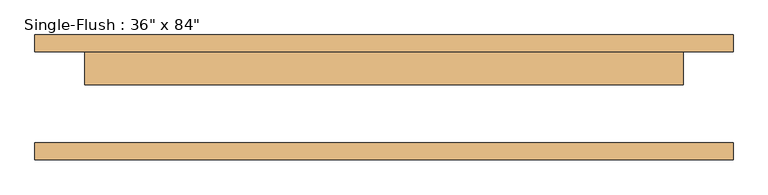
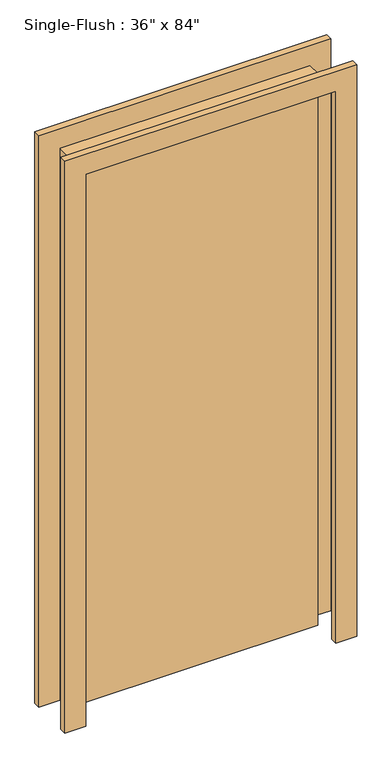
"""IFC4 building model written with IfcOpenShell, lengths in millimetres: door geometry."""

from ifc_helpers import new_model, si_unit, frame, origin, origin_with_axes, place, context, project, spatial, polyline, outline, extrude, source, transform, mapped, element, save


def door_c6edcd30(model_context):
    return source(origin(), model_context, "Body", "SweptSolid", [
        extrude(outline(polyline([(2209.8, -533.4), (0.0, -533.4), (0.0, -457.2), (2133.6, -457.2), (2133.6, 457.2), (0.0, 457.2), (0.0, 533.4), (2209.8, 533.4), (2209.8, -533.4)])), frame((0.0, 69.85, 0.0), z_axis=(0.0, 1.0, 0.0), x_axis=(0.0, 0.0, 1.0)), (0.0, 0.0, 1.0), 25.4),
        extrude(outline(polyline([(2209.8, 533.4), (2209.8, -533.4), (0.0, -533.4), (0.0, -457.2), (2133.6, -457.2), (2133.6, 457.2), (0.0, 457.2), (0.0, 533.4), (2209.8, 533.4)])), frame((0.0, -95.25, 0.0), z_axis=(0.0, 1.0, 0.0), x_axis=(0.0, 0.0, 1.0)), (0.0, 0.0, 1.0), 25.4),
        extrude(outline(polyline([(457.2, 19.05), (-457.2, 19.05), (-457.2, 69.85), (457.2, 69.85), (457.2, 19.05)])), origin_with_axes(), (0.0, 0.0, 1.0), 2133.6),
    ])


if __name__ == "__main__":
    model = new_model("IFC4")
    model_context = context("Model", 3, world=origin())
    ifc_project = project(units=[si_unit("LENGTHUNIT", "METRE", prefix="MILLI")], contexts=[model_context])
    site = spatial("IfcSite", under=ifc_project)
    building = spatial("IfcBuilding", under=site)
    placement = place(None, origin())
    door_shape = door_c6edcd30(model_context)
    element("IfcDoor", 1, ObjectType="Single-Flush : 36\" x 84\"", at=placement, inside=building, context=model_context, shape_type="MappedRepresentation", body=[
        mapped(door_shape, transform((0.0, 0.0, 0.0), x_axis=(1.0, 0.0, 0.0), y_axis=(0.0, 1.0, 0.0), z_axis=(0.0, 0.0, 1.0))),
    ])
    save(model, "model.ifc")

# Revit data of these elements
# Type "Single-Flush : 36\" x 84\""
#   Type Mark = "29"
#   Assembly Code = "C1020"
#   Thickness = 0' - 2"
#   Height = 7' - 0"
#   Trim Projection Ext = 0' - 1"
#   Trim Projection Int = 0' - 1"
#   Trim Width = 0' - 3"
#   Width = 3' - 0"
#   Function = 0
#   Door Material = Door - Panel
#   Frame Material = Concrete - Cast-in-Place Concrete
#   Wall Closure = (empty or 0)
# Element 1 (IfcDoor, "Single-Flush : 36\" x 84\"")
#   Materials on its faces: "Concrete - Cast-in-Place Concrete", "Door - Panel"
# Materials
#   "Door - Panel": class "Wood", colour RGB 149 143 132, transparency 0, Comments = "Rendering appearance not upgraded Rendering appearance not upgraded "
#   "Concrete - Cast-in-Place Concrete": class "Concrete", colour RGB 178 178 178, transparency 0, Comments = "Rendering appearance not upgraded Rendering appearance not upgraded ", Description = "Concrete"
